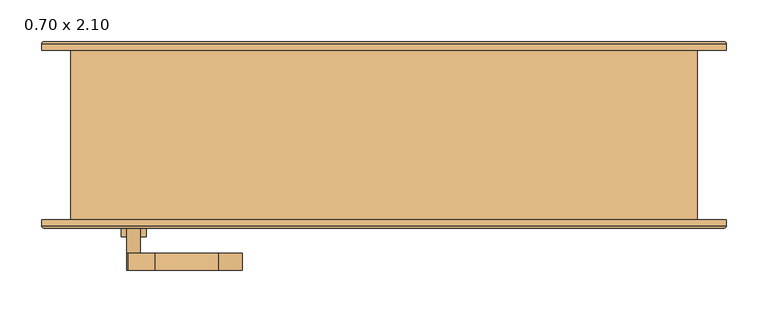
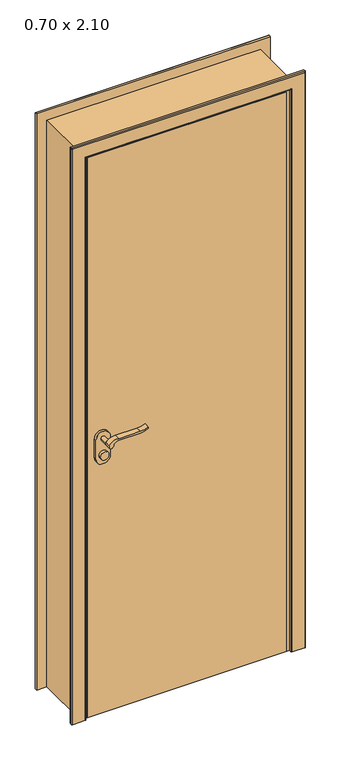
"""IFC4 building model written with IfcOpenShell, lengths in millimetres: door geometry, .CC_ND 300_PORTA SIMPLES DE ABRIR_COM EXTENSÃO : 0.70 x 2.10."""

import ifcopenshell
import ifcopenshell.guid

model = None  # the IFC model being written
_history = None  # IfcOwnerHistory: only IFC2X3 demands one
_inside = {}  # id of a spatial element -> (the spatial element, [elements in it])
_under = {}  # id of a project, library or spatial element -> (it, [spatial elements below it])
_declared = {}  # id of a project -> (the project, [libraries it declares])
_typed = {}  # id of a type object -> (the type object, [elements of that type])
_made_of = {}  # id of a material, layer set ... -> (it, [elements and type objects made of it])


def new_model(schema):
    """Start an empty IFC model of exactly this schema.

    Asked for "IFC4X3", IfcOpenShell would pick the latest addendum, in which some entities
    have other attributes; the version numbers below select the first issue.
    IFC2X3 requires an IfcOwnerHistory on every rooted entity: one is made here for all.
    """
    global model, _history
    if schema == "IFC4X3":
        model = ifcopenshell.file(schema_version=(4, 3, 0, 0))
    else:
        model = ifcopenshell.file(schema=schema)
    _inside.clear()
    _under.clear()
    _declared.clear()
    _typed.clear()
    _made_of.clear()
    _history = None
    if model.schema == "IFC2X3":
        org = make("IfcOrganization", Name="unknown")
        user = make(
            "IfcPersonAndOrganization",
            ThePerson=make("IfcPerson", FamilyName="unknown"),
            TheOrganization=org,
        )
        app = make(
            "IfcApplication",
            ApplicationDeveloper=org,
            Version="unknown",
            ApplicationFullName="unknown",
            ApplicationIdentifier="unknown",
        )
        _history = make(
            "IfcOwnerHistory",
            OwningUser=user,
            OwningApplication=app,
            ChangeAction="ADDED",
            CreationDate=0,
        )
    return model


def make(cls, **values):
    """One entity of the class cls with the attributes given. An attribute that is None is left unset."""
    return model.create_entity(
        cls, **{name: value for name, value in values.items() if value is not None}
    )


def rooted(cls, **values):
    """An entity with a GlobalId (a new one), such as an element, a storey or a relation."""
    return make(cls, GlobalId=ifcopenshell.guid.new(), OwnerHistory=_history, **values)


def si_unit(unit_type, name, prefix=None):
    """IfcSIUnit, for example si_unit("LENGTHUNIT", "METRE", prefix="MILLI")."""
    return make("IfcSIUnit", UnitType=unit_type, Prefix=prefix, Name=name)


def assignment(units):
    """IfcUnitAssignment: the units of a project."""
    return None if units is None else make("IfcUnitAssignment", Units=units)


def point(xyz):
    """IfcCartesianPoint."""
    return None if xyz is None else make("IfcCartesianPoint", Coordinates=xyz)


def direction(xyz):
    """IfcDirection."""
    return None if xyz is None else make("IfcDirection", DirectionRatios=xyz)


def frame(location, z_axis=None, x_axis=None):
    """IfcAxis2Placement3D, a coordinate frame: its origin and axes. An axis left out is left unset."""
    return make(
        "IfcAxis2Placement3D",
        Location=point(location),
        Axis=direction(z_axis),
        RefDirection=direction(x_axis),
    )


def frame_2d(location, x_axis=None):
    """IfcAxis2Placement2D, a coordinate frame in the plane: its origin and x axis."""
    return make(
        "IfcAxis2Placement2D", Location=point(location), RefDirection=direction(x_axis)
    )


def origin():
    """The frame at (0, 0, 0) with its axes left unset."""
    return frame((0.0, 0.0, 0.0))


def origin_with_axes():
    """The frame at (0, 0, 0) with the z axis (0, 0, 1) and the x axis (1, 0, 0) written out."""
    return frame((0.0, 0.0, 0.0), z_axis=(0.0, 0.0, 1.0), x_axis=(1.0, 0.0, 0.0))


def place(relative_to, where):
    """IfcLocalPlacement: puts the frame where relative to a parent placement (None: the world)."""
    return make(
        "IfcLocalPlacement", PlacementRelTo=relative_to, RelativePlacement=where
    )


def context(
    kind, dimensions, precision=None, world=None, true_north=None, identifier=None
):
    """IfcGeometricRepresentationContext, for example the 3D "Model" context."""
    return make(
        "IfcGeometricRepresentationContext",
        ContextIdentifier=identifier,
        ContextType=kind,
        CoordinateSpaceDimension=dimensions,
        Precision=precision,
        WorldCoordinateSystem=world,
        TrueNorth=true_north,
    )


def project(units=None, contexts=None):
    """IfcProject with its units and contexts."""
    return rooted(
        "IfcProject",
        Name="project",
        RepresentationContexts=contexts,
        UnitsInContext=assignment(units),
    )


def spatial(cls, under=None, at=None, **own):
    """A site, building, storey or space (cls), placed at a placement, below another one or the project."""
    s = rooted(cls, ObjectPlacement=at, **own)
    if under is not None:
        _under.setdefault(under.id(), (under, []))[1].append(s)
    return s


def polyline(points):
    """IfcPolyline through the points."""
    return make("IfcPolyline", Points=[point(p) for p in points])


def circle_curve(where, radius):
    """IfcCircle in the frame where."""
    return make("IfcCircle", Position=where, Radius=radius)


def ellipse_curve(where, semi_axis1, semi_axis2):
    """IfcEllipse in the frame where."""
    return make(
        "IfcEllipse", Position=where, SemiAxis1=semi_axis1, SemiAxis2=semi_axis2
    )


def trimmed(basis, trim1, trim2, sense, master):
    """IfcTrimmedCurve: the piece of a basis curve between two trims."""
    return make(
        "IfcTrimmedCurve",
        BasisCurve=basis,
        Trim1=trim1,
        Trim2=trim2,
        SenseAgreement=sense,
        MasterRepresentation=master,
    )


def segment(curve, same_sense, transition):
    """IfcCompositeCurveSegment."""
    return make(
        "IfcCompositeCurveSegment",
        Transition=transition,
        SameSense=same_sense,
        ParentCurve=curve,
    )


def composite_curve(segments, self_intersect=None):
    """IfcCompositeCurve: segments joined end to end."""
    return make("IfcCompositeCurve", Segments=segments, SelfIntersect=self_intersect)


def outline(outer, holes=None, kind="AREA"):
    """IfcArbitraryClosedProfileDef: a profile drawn as a closed curve; with holes, ...WithVoids."""
    if holes is None:
        return make("IfcArbitraryClosedProfileDef", ProfileType=kind, OuterCurve=outer)
    return make(
        "IfcArbitraryProfileDefWithVoids",
        ProfileType=kind,
        OuterCurve=outer,
        InnerCurves=holes,
    )


def extrude(swept, where, along, depth):
    """IfcExtrudedAreaSolid: the profile swept, set in the frame where, extruded along a direction by depth."""
    return make(
        "IfcExtrudedAreaSolid",
        SweptArea=swept,
        Position=where,
        ExtrudedDirection=direction(along),
        Depth=depth,
    )


def faces_of(points, faces, orient=None, outer=None):
    """IfcFace entities. A face is a list of loops; a loop is a list of indices into points, from 0.

    orient and outer hold one flag for each loop. By default every Orientation is true, the
    first loop of a face is its IfcFaceOuterBound and the others are IfcFaceBound.
    """
    made = []
    for i, loops in enumerate(faces):
        bounds = []
        for j, loop in enumerate(loops):
            is_outer = j == 0 if outer is None else outer[i][j]
            bounds.append(
                make(
                    "IfcFaceOuterBound" if is_outer else "IfcFaceBound",
                    Bound=make("IfcPolyLoop", Polygon=[points[k] for k in loop]),
                    Orientation=True if orient is None else orient[i][j],
                )
            )
        made.append(make("IfcFace", Bounds=bounds))
    return made


def faceted_brep(points, faces, orient=None, outer=None, voids=None):
    """IfcFacetedBrep: a solid bounded by flat faces; with voids (closed shells), ...WithVoids."""
    shared = [point(p) for p in points]
    hull = make("IfcClosedShell", CfsFaces=faces_of(shared, faces, orient, outer))
    if voids is None:
        return make("IfcFacetedBrep", Outer=hull)
    return make(
        "IfcFacetedBrepWithVoids",
        Outer=hull,
        Voids=[
            make(cls, CfsFaces=faces_of(shared, fs, o, b)) for cls, fs, o, b in voids
        ],
    )


def shape(context_of_items, identifier, shape_type, items):
    """IfcShapeRepresentation: the items that make up one representation, for example the "Body"."""
    return make(
        "IfcShapeRepresentation",
        ContextOfItems=context_of_items,
        RepresentationIdentifier=identifier,
        RepresentationType=shape_type,
        Items=items,
    )


def source(mapping_origin, context_of_items, identifier, shape_type, items):
    """IfcRepresentationMap: a shape defined once, which mapped items show again and again."""
    return make(
        "IfcRepresentationMap",
        MappingOrigin=mapping_origin,
        MappedRepresentation=shape(context_of_items, identifier, shape_type, items),
    )


def transform(
    local_origin,
    x_axis=None,
    y_axis=None,
    z_axis=None,
    scale=None,
    scale2=None,
    scale3=None,
    uniform=True,
):
    """IfcCartesianTransformationOperator3D, or its non-uniform kind. x_axis, y_axis, z_axis: its Axis1, 2, 3."""
    if uniform:
        return make(
            "IfcCartesianTransformationOperator3D",
            Axis1=direction(x_axis),
            Axis2=direction(y_axis),
            LocalOrigin=point(local_origin),
            Scale=scale,
            Axis3=direction(z_axis),
        )
    return make(
        "IfcCartesianTransformationOperator3DnonUniform",
        Axis1=direction(x_axis),
        Axis2=direction(y_axis),
        LocalOrigin=point(local_origin),
        Scale=scale,
        Axis3=direction(z_axis),
        Scale2=scale2,
        Scale3=scale3,
    )


def mapped(mapping_source, mapping_target):
    """IfcMappedItem: shows the shape of a source again, moved by a transform."""
    return make(
        "IfcMappedItem", MappingSource=mapping_source, MappingTarget=mapping_target
    )


def made_of(thing, what):
    """Note that an element or type object is made of a material, layer set ...; save() writes the relation."""
    if what is not None:
        _made_of.setdefault(what.id(), (what, []))[1].append(thing)
    return thing


def element(
    cls,
    number,
    at=None,
    inside=None,
    cuts=None,
    type_object=None,
    material=None,
    context=None,
    identifier="Body",
    shape_type=None,
    held_by="IfcProductDefinitionShape",
    body=None,
    shapes=None,
    **own,
):
    """One element of the class cls, such as IfcWall. Its Tag is "e" and its number.

    at: its placement. inside: the storey or other place that contains it. cuts: it is an
    opening in that element (IfcRelVoidsElement). A single representation is given by context,
    identifier, shape_type and body (its items); several are given by shapes. held_by: the class
    of the entity that holds the representations. save() writes the other relations.
    """
    e = rooted(cls, Tag="e%d" % number, ObjectPlacement=at, **own)
    if body is not None:
        shapes = [shape(context, identifier, shape_type, body)]
    if shapes is not None:
        e.Representation = make(held_by, Representations=shapes)
    if inside is not None:
        _inside.setdefault(inside.id(), (inside, []))[1].append(e)
    if cuts is not None:
        rooted(
            "IfcRelVoidsElement", RelatingBuildingElement=cuts, RelatedOpeningElement=e
        )
    if type_object is not None:
        _typed.setdefault(type_object.id(), (type_object, []))[1].append(e)
    return made_of(e, material)


def aggregate(whole, parts):
    """IfcRelAggregates: a whole, such as a stair, and the parts it consists of."""
    return rooted("IfcRelAggregates", RelatingObject=whole, RelatedObjects=parts)


def save(model, path):
    """Write the relations noted so far, then the file.

    IfcRelAggregates (storeys below a building ...), IfcRelContainedInSpatialStructure (elements
    in a storey), IfcRelDefinesByType, IfcRelAssociatesMaterial and IfcRelDeclares: one each for
    every whole, place, type object, material and project.
    """
    for whole, parts in _under.values():
        aggregate(whole, parts)
    for where, things in _inside.values():
        rooted(
            "IfcRelContainedInSpatialStructure",
            RelatedElements=things,
            RelatingStructure=where,
        )
    for kind, things in _typed.values():
        rooted("IfcRelDefinesByType", RelatedObjects=things, RelatingType=kind)
    for what, things in _made_of.values():
        rooted("IfcRelAssociatesMaterial", RelatedObjects=things, RelatingMaterial=what)
    for by, libraries in _declared.values():
        rooted("IfcRelDeclares", RelatingContext=by, RelatedDefinitions=libraries)
    model.write(path)


def plane_surface(at):
    """IfcPlane: the flat surface through the origin of the frame at, square to its z axis."""
    return make("IfcPlane", Position=at)


def cylinder_surface(at, radius):
    """IfcCylindricalSurface: all points at the distance radius from the z axis of the frame at."""
    return make("IfcCylindricalSurface", Position=at, Radius=radius)


def advanced_brep(points, edges, surfaces, faces):
    """IfcAdvancedBrep: a solid bounded by faces that lie on surfaces and meet in shared edges.

    An edge is (start, end): straight between two places in points (the first is 0);
    or (start, end, curve); or (start, end, curve, False) where it runs against its curve.
    A face is (place in surfaces, loops), or (place, loops, False) where it looks against
    its surface's normal. A loop lists edges by number (the first is 1), with a minus sign
    where the edge is run from its end to its start. The first loop is the outer one.
    """
    corners = [point(p) for p in points]
    vertices = [make("IfcVertexPoint", VertexGeometry=c) for c in corners]
    made = []
    for start, end, *more in edges:
        made.append(
            make(
                "IfcEdgeCurve",
                EdgeStart=vertices[start],
                EdgeEnd=vertices[end],
                EdgeGeometry=more[0] if more else make("IfcPolyline", Points=[corners[start], corners[end]]),
                SameSense=more[1] if len(more) > 1 else True,
            )
        )
    hull = []
    for where, loops, *sense in faces:
        bounds = []
        for j, loop in enumerate(loops):
            ring = [make("IfcOrientedEdge", EdgeElement=made[abs(k) - 1], Orientation=k > 0) for k in loop]
            bounds.append(
                make(
                    "IfcFaceOuterBound" if j == 0 else "IfcFaceBound",
                    Bound=make("IfcEdgeLoop", EdgeList=ring),
                    Orientation=True,
                )
            )
        hull.append(make("IfcAdvancedFace", Bounds=bounds, FaceSurface=surfaces[where], SameSense=sense[0] if sense else True))
    return make("IfcAdvancedBrep", Outer=make("IfcClosedShell", CfsFaces=hull))


def door_0_70_x_2_10_0ff34c02(model_context):
    return source(origin(), model_context, "Body", "SolidModel", [
        extrude(outline(composite_curve([segment(trimmed(circle_curve(frame_2d((964.5, -300.0)), 15.0), [point((964.5, -285.0))], [point((964.5, -315.0))], False, "CARTESIAN"), True, "CONTINUOUS"), segment(trimmed(circle_curve(frame_2d((964.5, -300.0)), 15.0), [point((964.5, -315.0))], [point((964.5, -285.0))], False, "CARTESIAN"), True, "CONTINUOUS")], self_intersect=False)), frame((0.0, -136.4, 0.0), z_axis=(0.0, 1.0, 0.0), x_axis=(0.0, 0.0, 1.0)), (0.0, 0.0, 1.0), 10.0),
        extrude(outline(composite_curve([segment(trimmed(circle_curve(frame_2d((964.5, -300.0)), 15.0), [point((964.5, -285.0))], [point((964.5, -315.0))], False, "CARTESIAN"), True, "CONTINUOUS"), segment(trimmed(circle_curve(frame_2d((964.5, -300.0)), 15.0), [point((964.5, -315.0))], [point((964.5, -285.0))], False, "CARTESIAN"), True, "CONTINUOUS")], self_intersect=False)), frame((0.0, -76.4, 0.0), z_axis=(0.0, 1.0, 0.0), x_axis=(0.0, 0.0, 1.0)), (0.0, 0.0, 1.0), 10.0),
        extrude(outline(composite_curve([segment(trimmed(circle_curve(frame_2d((1024.5, -300.0)), 8.0), [point((1029.1523287, -306.5081363))], [point((1024.5, -292.0))], False, "CARTESIAN"), True, "CONTINUOUS"), segment(trimmed(circle_curve(frame_2d((1019.3738613, -274.6138099)), 18.1261387), [point((1024.5, -292.0))], [point((1037.5, -274.6138099))], True, "CARTESIAN"), True, "CONTINUOUS"), segment(polyline([(1037.5, -274.6138099), (1037.5, -198.3564091)]), True, "CONTINUOUS"), segment(trimmed(circle_curve(frame_2d((1096.7709207, -201.9396612)), 59.3791355), [point((1037.5, -198.3564091))], [point((1046.7135558, -170.0))], False, "CARTESIAN"), True, "CONTINUOUS"), segment(polyline([(1046.7135558, -170.0), (1049.5, -170.0)]), True, "CONTINUOUS"), segment(trimmed(circle_curve(frame_2d((1127.7850638, -198.4227909)), 83.2850902), [point((1049.5, -170.0))], [point((1044.5, -198.3564091))], True, "CARTESIAN"), True, "CONTINUOUS"), segment(polyline([(1044.5, -198.3564091), (1044.5, -274.6325667)]), True, "CONTINUOUS"), segment(trimmed(circle_curve(frame_2d((1007.2555521, -276.3324871)), 37.2832219), [point((1044.5, -274.6325667))], [point((1029.1523287, -306.5081363))], False, "CARTESIAN"), True, "CONTINUOUS")], self_intersect=False)), frame((0.0, -176.4, 0.0), z_axis=(0.0, 1.0, 0.0), x_axis=(0.0, 0.0, 1.0)), (0.0, 0.0, 1.0), 20.0),
        extrude(outline(composite_curve([segment(trimmed(circle_curve(frame_2d((1019.3738682, -274.6138122)), 18.1261318), [point((1024.4999903, -292.0))], [point((1037.5, -274.6138122))], True, "CARTESIAN"), True, "CONTINUOUS"), segment(polyline([(1037.5, -274.6138122), (1037.5, -198.3564091)]), True, "CONTINUOUS"), segment(trimmed(circle_curve(frame_2d((1096.7709207, -201.9396612)), 59.3791355), [point((1037.5, -198.3564091))], [point((1046.7135558, -170.0))], False, "CARTESIAN"), True, "CONTINUOUS"), segment(polyline([(1046.7135558, -170.0), (1049.5, -170.0)]), True, "CONTINUOUS"), segment(trimmed(circle_curve(frame_2d((1127.7850638, -198.4227909)), 83.2850902), [point((1049.5, -170.0))], [point((1044.5, -198.3564091))], True, "CARTESIAN"), True, "CONTINUOUS"), segment(polyline([(1044.5, -198.3564091), (1044.5, -274.6325667)]), True, "CONTINUOUS"), segment(trimmed(circle_curve(frame_2d((1007.2555521, -276.3324871)), 37.2832219), [point((1044.5, -274.6325667))], [point((1029.1523287, -306.5081363))], False, "CARTESIAN"), True, "CONTINUOUS"), segment(trimmed(circle_curve(frame_2d((1024.5, -300.0)), 8.0), [point((1029.1523287, -306.5081363))], [point((1024.4999903, -292.0))], False, "CARTESIAN"), True, "CONTINUOUS")], self_intersect=False)), frame((0.0, -46.4, 0.0), z_axis=(0.0, 1.0, 0.0), x_axis=(0.0, 0.0, 1.0)), (0.0, 0.0, 1.0), 20.0),
        extrude(outline(composite_curve([segment(trimmed(circle_curve(frame_2d((1024.5, -300.0)), 8.0), [point((1024.5, -292.0))], [point((1024.5, -308.0))], False, "CARTESIAN"), True, "CONTINUOUS"), segment(trimmed(circle_curve(frame_2d((1024.5, -300.0)), 8.0), [point((1024.5, -308.0))], [point((1024.5, -292.0))], False, "CARTESIAN"), True, "CONTINUOUS")], self_intersect=False)), frame((0.0, -156.4, 0.0), z_axis=(0.0, 1.0, 0.0), x_axis=(0.0, 0.0, 1.0)), (0.0, 0.0, 1.0), 30.0),
        extrude(outline(composite_curve([segment(trimmed(circle_curve(frame_2d((1024.5, -300.0)), 8.0), [point((1024.5, -292.0))], [point((1024.5, -308.0))], False, "CARTESIAN"), True, "CONTINUOUS"), segment(trimmed(circle_curve(frame_2d((1024.5, -300.0)), 8.0), [point((1024.5, -308.0))], [point((1024.5, -292.0))], False, "CARTESIAN"), True, "CONTINUOUS")], self_intersect=False)), frame((0.0, -76.4, 0.0), z_axis=(0.0, 1.0, 0.0), x_axis=(0.0, 0.0, 1.0)), (0.0, 0.0, 1.0), 30.0),
        extrude(outline(composite_curve([segment(trimmed(circle_curve(frame_2d((954.5, -300.0)), 25.0), [point((954.5, -325.0))], [point((954.5, -275.0))], False, "CARTESIAN"), True, "CONTINUOUS"), segment(polyline([(954.5, -275.0), (1024.5, -275.0)]), True, "CONTINUOUS"), segment(trimmed(circle_curve(frame_2d((1024.5, -300.0)), 25.0), [point((1024.5, -275.0))], [point((1024.5, -325.0))], False, "CARTESIAN"), True, "CONTINUOUS"), segment(polyline([(1024.5, -325.0), (954.5, -325.0)]), True, "CONTINUOUS")], self_intersect=False)), frame((0.0, -126.4, 0.0), z_axis=(0.0, 1.0, 0.0), x_axis=(0.0, 0.0, 1.0)), (0.0, 0.0, 1.0), 10.0),
        extrude(outline(composite_curve([segment(trimmed(circle_curve(frame_2d((954.5, -300.0)), 25.0), [point((954.5, -325.0))], [point((954.5, -275.0))], False, "CARTESIAN"), True, "CONTINUOUS"), segment(polyline([(954.5, -275.0), (1024.5, -275.0)]), True, "CONTINUOUS"), segment(trimmed(circle_curve(frame_2d((1024.5, -300.0)), 25.0), [point((1024.5, -275.0))], [point((1024.5, -325.0))], False, "CARTESIAN"), True, "CONTINUOUS"), segment(polyline([(1024.5, -325.0), (954.5, -325.0)]), True, "CONTINUOUS")], self_intersect=False)), frame((0.0, -86.4, 0.0), z_axis=(0.0, 1.0, 0.0), x_axis=(0.0, 0.0, 1.0)), (0.0, 0.0, 1.0), 10.0),
        advanced_brep(
        [(-410.0, -116.4, 0.0), (-360.0, -116.4, 0.0), (-360.0, -123.4, 0.0), (-363.0, -126.4, 0.0), (-407.0, -126.4, 0.0), (-410.0, -123.4, 0.0), (-410.0, -116.4, 2135.0), (410.0, -116.4, 2135.0), (410.0, -116.4, 0.0), (360.0, -116.4, 0.0), (360.0, -116.4, 2085.0), (-360.0, -116.4, 2085.0), (-360.0, -123.4, 2085.0), (-363.0, -126.4, 2088.0), (363.0, -126.4, 2088.0), (363.0, -126.4, 0.0), (407.0, -126.4, 0.0), (407.0, -126.4, 2132.0), (-407.0, -126.4, 2132.0), (-410.0, -123.4, 2135.0), (410.0, -123.4, 2135.0), (410.0, -123.4, 0.0), (360.0, -123.4, 0.0), (360.0, -123.4, 2085.0)],
        [
            (0, 1),
            (1, 2),
            (2, 3, circle_curve(frame((-363.0, -123.4, 0.0), z_axis=(0.0, 0.0, -1.0), x_axis=(1.0, 0.0, 0.0)), 3.0)),
            (3, 4),
            (4, 5, circle_curve(frame((-407.0, -123.4, 0.0), z_axis=(0.0, 0.0, -1.0), x_axis=(1.0, 0.0, 0.0)), 3.0)),
            (5, 0),
            (0, 6),
            (6, 7),
            (7, 8),
            (8, 9),
            (9, 10),
            (10, 11),
            (11, 1),
            (11, 12),
            (12, 2),
            (12, 13, ellipse_curve(frame((-363.0, -123.4, 2088.0), z_axis=(-0.7071067811865475, 0.0, -0.7071067811865475), x_axis=(0.7071067811865474, 0.0, -0.7071067811865476)), 4.2426407, 3.0)),
            (13, 3),
            (13, 14),
            (14, 15),
            (15, 16),
            (16, 17),
            (17, 18),
            (18, 4),
            (18, 19, ellipse_curve(frame((-407.0, -123.4, 2132.0), z_axis=(-0.7071067811865475, 0.0, -0.7071067811865475), x_axis=(0.7071067811865474, 0.0, -0.7071067811865476)), 4.2426407, 3.0)),
            (19, 5),
            (19, 6),
            (7, 20),
            (20, 21),
            (21, 8),
            (21, 16, circle_curve(frame((407.0, -123.4, 0.0), z_axis=(0.0, 0.0, -1.0), x_axis=(-1.0, 0.0, 0.0)), 3.0)),
            (15, 22, circle_curve(frame((363.0, -123.4, 0.0), z_axis=(0.0, 0.0, -1.0), x_axis=(-1.0, 0.0, 0.0)), 3.0)),
            (22, 9),
            (23, 10),
            (22, 23),
            (14, 23, ellipse_curve(frame((363.0, -123.4, 2088.0), z_axis=(0.7071067811865475, 0.0, -0.7071067811865475), x_axis=(0.7071067811865474, 0.0, 0.7071067811865476)), 4.2426407, 3.0)),
            (20, 17, ellipse_curve(frame((407.0, -123.4, 2132.0), z_axis=(0.7071067811865475, 0.0, -0.7071067811865475), x_axis=(0.7071067811865474, 0.0, 0.7071067811865476)), 4.2426407, 3.0)),
            (23, 12),
            (19, 20),
        ],
        [
            plane_surface(frame((-360.0, -116.4, 0.0), z_axis=(0.0, 0.0, -1.0), x_axis=(0.0, 1.0, 0.0))),
            plane_surface(frame((-410.0, -116.4, 0.0), z_axis=(0.0, 1.0, 0.0), x_axis=(0.0, 0.0, 1.0))),
            plane_surface(frame((-360.0, -116.4, 0.0), z_axis=(1.0, 0.0, 0.0), x_axis=(0.0, 0.0, 1.0))),
            cylinder_surface(frame((-363.0, -123.4, 0.0), z_axis=(0.0, 0.0, -1.0), x_axis=(1.0, 0.0, 0.0)), 3.0),
            plane_surface(frame((-363.0, -126.4, 0.0), z_axis=(0.0, -1.0, 0.0), x_axis=(0.0, 0.0, 1.0))),
            cylinder_surface(frame((-407.0, -123.4, 0.0), z_axis=(0.0, 0.0, -1.0), x_axis=(1.0, 0.0, 0.0)), 3.0),
            plane_surface(frame((-410.0, -123.4, 0.0), z_axis=(-1.0, 0.0, 0.0), x_axis=(0.0, 0.0, 1.0))),
            plane_surface(frame((410.0, -123.4, 2135.0), z_axis=(1.0, 0.0, 0.0), x_axis=(0.0, 0.0, -1.0))),
            plane_surface(frame((360.0, -116.4, 0.0), z_axis=(0.0, 0.0, -1.0), x_axis=(0.0, 1.0, 0.0))),
            plane_surface(frame((360.0, -116.4, 2085.0), z_axis=(-1.0, 0.0, 0.0), x_axis=(0.0, 0.0, -1.0))),
            cylinder_surface(frame((363.0, -123.4, 2085.0), z_axis=(0.0, 0.0, 1.0), x_axis=(-1.0, 0.0, 0.0)), 3.0),
            cylinder_surface(frame((407.0, -123.4, 2085.0), z_axis=(0.0, 0.0, 1.0), x_axis=(-1.0, 0.0, 0.0)), 3.0),
            plane_surface(frame((-360.0, -116.4, 2085.0), z_axis=(0.0, 0.0, -1.0), x_axis=(1.0, 0.0, 0.0))),
            plane_surface(frame((-410.0, -123.4, 2135.0), z_axis=(0.0, 0.0, 1.0), x_axis=(1.0, 0.0, 0.0))),
            cylinder_surface(frame((-360.0, -123.4, 2088.0), z_axis=(-1.0, 0.0, 0.0), x_axis=(0.0, 0.0, -1.0)), 3.0),
            cylinder_surface(frame((-360.0, -123.4, 2132.0), z_axis=(-1.0, 0.0, 0.0), x_axis=(0.0, 0.0, -1.0)), 3.0),
        ],
        [
            (0, [[1, 2, 3, 4, 5, 6]]),
            (1, [[-1, 7, 8, 9, 10, 11, 12, 13]]),
            (2, [[-2, -13, 14, 15]]),
            (3, [[-3, -15, 16, 17]]),
            (4, [[-4, -17, 18, 19, 20, 21, 22, 23]]),
            (5, [[-5, -23, 24, 25]]),
            (6, [[-6, -25, 26, -7]]),
            (7, [[27, 28, 29, -9]]),
            (8, [[-29, 30, -20, 31, 32, -10]]),
            (9, [[33, -11, -32, 34]]),
            (10, [[35, -34, -31, -19]]),
            (11, [[36, -21, -30, -28]]),
            (12, [[-14, -12, -33, 37]]),
            (13, [[-26, 38, -27, -8]]),
            (14, [[-16, -37, -35, -18]]),
            (15, [[-24, -22, -36, -38]]),
        ],
    ),
        advanced_brep(
        [(410.0, 86.9, 0.0), (360.0, 86.9, 0.0), (360.0, 93.9157283, 0.0), (362.9842717, 96.9, 0.0), (407.0342217, 96.9, 0.0), (410.0, 93.9342217, 0.0), (410.0, 86.9, 2135.0), (-410.0, 86.9, 2135.0), (-410.0, 86.9, 0.0), (-360.0, 86.9, 0.0), (-360.0, 86.9, 2085.0), (360.0, 86.9, 2085.0), (360.0, 93.9157283, 2085.0), (362.9842717, 96.9, 2087.9842717), (-362.9842717, 96.9, 2087.9842717), (-362.9842717, 96.9, 0.0), (-407.0342217, 96.9, 0.0), (-407.0342217, 96.9, 2132.0342217), (407.0342217, 96.9, 2132.0342217), (410.0, 93.9342217, 2135.0), (-410.0, 93.9342217, 2135.0), (-410.0, 93.9342217, 0.0), (-360.0, 93.9157283, 0.0), (-360.0, 93.9157283, 2085.0)],
        [
            (0, 1),
            (1, 2),
            (2, 3, circle_curve(frame((362.9842717, 93.9157283, 0.0), z_axis=(0.0, 0.0, -1.0), x_axis=(1.0, 0.0, 0.0)), 2.9842717)),
            (3, 4),
            (4, 5, circle_curve(frame((407.0342217, 93.9342217, 0.0), z_axis=(0.0, 0.0, -1.0), x_axis=(1.0, 0.0, 0.0)), 2.9657783)),
            (5, 0),
            (0, 6),
            (6, 7),
            (7, 8),
            (8, 9),
            (9, 10),
            (10, 11),
            (11, 1),
            (11, 12),
            (12, 2),
            (12, 13, ellipse_curve(frame((362.9842717, 93.9157283, 2087.9842717), z_axis=(0.7071067811865475, 0.0, -0.7071067811865475), x_axis=(-0.7071067811865474, 0.0, -0.7071067811865476)), 4.2203975, 2.9842717)),
            (13, 3),
            (13, 14),
            (14, 15),
            (15, 16),
            (16, 17),
            (17, 18),
            (18, 4),
            (18, 19, ellipse_curve(frame((407.0342217, 93.9342217, 2132.0342217), z_axis=(0.7071067811865475, 0.0, -0.7071067811865475), x_axis=(-0.7071067811865474, 0.0, -0.7071067811865476)), 4.1942438, 2.9657783)),
            (19, 5),
            (19, 6),
            (7, 20),
            (20, 21),
            (21, 8),
            (21, 16, circle_curve(frame((-407.0342217, 93.9342217, 0.0), z_axis=(0.0, 0.0, -1.0), x_axis=(-1.0, 0.0, 0.0)), 2.9657783)),
            (15, 22, circle_curve(frame((-362.9842717, 93.9157283, 0.0), z_axis=(0.0, 0.0, -1.0), x_axis=(-1.0, 0.0, 0.0)), 2.9842717)),
            (22, 9),
            (23, 10),
            (22, 23),
            (14, 23, ellipse_curve(frame((-362.9842717, 93.9157283, 2087.9842717), z_axis=(-0.7071067811865475, 0.0, -0.7071067811865475), x_axis=(-0.7071067811865474, 0.0, 0.7071067811865476)), 4.2203975, 2.9842717)),
            (20, 17, ellipse_curve(frame((-407.0342217, 93.9342217, 2132.0342217), z_axis=(-0.7071067811865475, 0.0, -0.7071067811865475), x_axis=(-0.7071067811865474, 0.0, 0.7071067811865476)), 4.1942438, 2.9657783)),
            (23, 12),
            (19, 20),
        ],
        [
            plane_surface(frame((360.0, 86.9, 0.0), z_axis=(0.0, 0.0, -1.0), x_axis=(0.0, 1.0, 0.0))),
            plane_surface(frame((410.0, 86.9, 0.0), z_axis=(0.0, -1.0, 0.0), x_axis=(0.0, 0.0, 1.0))),
            plane_surface(frame((360.0, 86.9, 0.0), z_axis=(-1.0, 0.0, 0.0), x_axis=(0.0, 0.0, 1.0))),
            cylinder_surface(frame((362.9842717, 93.9157283, 0.0), z_axis=(0.0, 0.0, -1.0), x_axis=(1.0, 0.0, 0.0)), 2.9842717),
            plane_surface(frame((362.9842717, 96.9, 0.0), z_axis=(0.0, 1.0, 0.0), x_axis=(0.0, 0.0, 1.0))),
            cylinder_surface(frame((407.0342217, 93.9342217, 0.0), z_axis=(0.0, 0.0, -1.0), x_axis=(1.0, 0.0, 0.0)), 2.9657783),
            plane_surface(frame((410.0, 93.9342217, 0.0), z_axis=(1.0, 0.0, 0.0), x_axis=(0.0, 0.0, 1.0))),
            plane_surface(frame((-410.0, 93.9342217, 2135.0), z_axis=(-1.0, 0.0, 0.0), x_axis=(0.0, 0.0, -1.0))),
            plane_surface(frame((-360.0, 86.9, 0.0), z_axis=(0.0, 0.0, -1.0), x_axis=(0.0, 1.0, 0.0))),
            plane_surface(frame((-360.0, 86.9, 2085.0), z_axis=(1.0, 0.0, 0.0), x_axis=(0.0, 0.0, -1.0))),
            cylinder_surface(frame((-362.9842717, 93.9157283, 2085.0), z_axis=(0.0, 0.0, 1.0), x_axis=(-1.0, 0.0, 0.0)), 2.9842717),
            cylinder_surface(frame((-407.0342217, 93.9342217, 2085.0), z_axis=(0.0, 0.0, 1.0), x_axis=(-1.0, 0.0, 0.0)), 2.9657783),
            plane_surface(frame((360.0, 86.9, 2085.0), z_axis=(0.0, 0.0, -1.0), x_axis=(-1.0, 0.0, 0.0))),
            plane_surface(frame((410.0, 93.9342217, 2135.0), z_axis=(0.0, 0.0, 1.0), x_axis=(-1.0, 0.0, 0.0))),
            cylinder_surface(frame((360.0, 93.9157283, 2087.9842717), z_axis=(1.0, 0.0, 0.0), x_axis=(0.0, 0.0, 1.0)), 2.9842717),
            cylinder_surface(frame((360.0, 93.9342217, 2132.0342217), z_axis=(1.0, 0.0, 0.0), x_axis=(0.0, 0.0, 1.0)), 2.9657783),
        ],
        [
            (0, [[1, 2, 3, 4, 5, 6]]),
            (1, [[-1, 7, 8, 9, 10, 11, 12, 13]]),
            (2, [[-2, -13, 14, 15]]),
            (3, [[-3, -15, 16, 17]]),
            (4, [[-4, -17, 18, 19, 20, 21, 22, 23]]),
            (5, [[-5, -23, 24, 25]]),
            (6, [[-6, -25, 26, -7]]),
            (7, [[27, 28, 29, -9]]),
            (8, [[-29, 30, -20, 31, 32, -10]]),
            (9, [[33, -11, -32, 34]]),
            (10, [[35, -34, -31, -19]]),
            (11, [[36, -21, -30, -28]]),
            (12, [[-14, -12, -33, 37]]),
            (13, [[-26, 38, -27, -8]]),
            (14, [[-16, -37, -35, -18]]),
            (15, [[-24, -22, -36, -38]]),
        ],
    ),
        faceted_brep([(342.0, 86.9, 0.0), (375.0, 86.9, 0.0), (375.0, -116.4, 0.0), (350.0, -116.4, 0.0), (350.0, -86.4, 0.0), (342.0, -86.4, 0.0), (342.0, 86.9, 2067.0), (-342.0, 86.9, 2067.0), (-342.0, 86.9, 0.0), (-375.0, 86.9, 0.0), (-375.0, 86.9, 2100.0), (375.0, 86.9, 2100.0), (375.0, -116.4, 2100.0), (-375.0, -116.4, 2100.0), (-375.0, -116.4, 0.0), (-350.0, -116.4, 0.0), (-350.0, -116.4, 2075.0), (350.0, -116.4, 2075.0), (350.0, -86.4, 2075.0), (-350.0, -86.4, 2075.0), (-350.0, -86.4, 0.0), (-342.0, -86.4, 0.0), (-342.0, -86.4, 2067.0), (342.0, -86.4, 2067.0)], [[[0, 1, 2, 3, 4, 5]], [[1, 0, 6, 7, 8, 9, 10, 11]], [[2, 1, 11, 12]], [[3, 2, 12, 13, 14, 15, 16, 17]], [[4, 3, 17, 18]], [[5, 4, 18, 19, 20, 21, 22, 23]], [[0, 5, 23, 6]], [[7, 22, 21, 8]], [[8, 21, 20, 15, 14, 9]], [[13, 10, 9, 14]], [[19, 16, 15, 20]], [[12, 11, 10, 13]], [[18, 17, 16, 19]], [[6, 23, 22, 7]]]),
        extrude(outline(polyline([(-350.0, -86.4), (350.0, -86.4), (350.0, -116.4), (-350.0, -116.4), (-350.0, -86.4)])), origin_with_axes(), (0.0, 0.0, 1.0), 2075.0),
    ])


if __name__ == "__main__":
    model = new_model("IFC4")
    model_context = context("Model", 3, world=origin())
    ifc_project = project(units=[si_unit("LENGTHUNIT", "METRE", prefix="MILLI")], contexts=[model_context])
    site = spatial("IfcSite", under=ifc_project)
    building = spatial("IfcBuilding", under=site)
    placement = place(None, origin())
    door_0_70_x_2_10_shape = door_0_70_x_2_10_0ff34c02(model_context)
    element("IfcDoor", 1, ObjectType=".CC_ND 300_PORTA SIMPLES DE ABRIR_COM EXTENSÃO : 0.70 x 2.10", at=placement, inside=building, context=model_context, shape_type="MappedRepresentation", body=[
        mapped(door_0_70_x_2_10_shape, transform((0.0, 0.0, 0.0), x_axis=(1.0, 0.0, 0.0), y_axis=(0.0, 1.0, 0.0), z_axis=(0.0, 0.0, 1.0))),
    ])
    save(model, "model.ifc")

# Revit data of these elements
# Project information
#   Design Option = "Main Model"
#   Project Status = "Status do projeto"
#   Project Address = "RUA SÉRGIO DIAS, LOTE 30, QUADRA G, MONTE MINEIRO/MG"
#   Project Name = "RESIDÊNCIA - ROBERTA VENDRAMINI"
#   Project Number = "034/2017"
#   Zona = "ZER - 01"
#   CA Mín = "0.2"
#   CA Básico = "1"
#   CA Máx = "2"
#   TO Máx = "50"
#   Gabarito Máx = "10"
#   TP Mín = "15"
#   Área Total do Terreno = "620.00 m²"
#   Multifamiliar - Vagas Veículos/Pavto = "0"
#   Multifamiliar - Vagas Bicicletas/Pavto = "0"
#   Multifamiliar - % Vagas PNMR = "0"
#   Multifamiliar - % Vagas Motos = "0"
#   Outros - Área p/ 1 Veículo = "0.00 m²"
#   Outros - Área p/ 1 Bicicleta = "0.00 m²"
#   Outros - Área p/ 1 Utilitário = "0.00 m²"
#   Outros - % Vagas PNMR = "0"
#   Outros - % Vagas Motos = "0"
# Type ".CC_ND 300_PORTA SIMPLES DE ABRIR_COM EXTENSÃO : 0.70 x 2.10"
#   Type Mark = "155"
#   Rough Width = 0.75 m
#   Espessura moldura externa = 0.01 m
#   Espessura moldura interna = 0.01 m
#   Largura moldura = 0.05 m
#   Extensão acabamento exterior [instance default] = 0.00 m
#   Extensão acabamento interior [instance default] = 0.00 m
#   Espessura batente = 0.025 m
#   Thickness = 0.03 m
#   Altura batente = 2.085 m
#   Aux Arco [instance default] = 0.70 m
#   Rough Height = 2.125 m
#   Height = 2.10 m
#   Width = 0.70 m
#   Moldura interna [instance default] = yes
#   Moldura externa [instance default] = yes
#   Porta = .MADEIRA COM PINTURA ESMALTE BRANCO ACETINADO
#   Moldura = .MADEIRA COM PINTURA ESMALTE BRANCO ACETINADO
#   Maçaneta = .ALUMÍNIO
#   Batente = .MADEIRA COM PINTURA ESMALTE BRANCO ACETINADO
#   Function = (empty or 0)
#   Wall Closure = (empty or 0)
# Element 1 (IfcDoor, ".CC_ND 300_PORTA SIMPLES DE ABRIR_COM EXTENSÃO : 0.70 x 2.10")
#   Extensão acabamento interior = 0.0295 m
#   Aux Arco = 0.7295 m
#   Materials on its faces: ".MADEIRA COM PINTURA ESMALTE BRANCO ACETINADO", ".ALUMÍNIO"
# Materials
#   ".MADEIRA COM PINTURA ESMALTE BRANCO ACETINADO": class ".CC_MADEIRAS", colour RGB 240 240 240, transparency 0, Description = "Madeira com pintura esmalte branco acetinado.", Cost = 0
#   ".ALUMÍNIO": class "CC_METAIS", colour RGB 244 244 244, transparency 0, Description = "Material alumínio", Cost = 0
